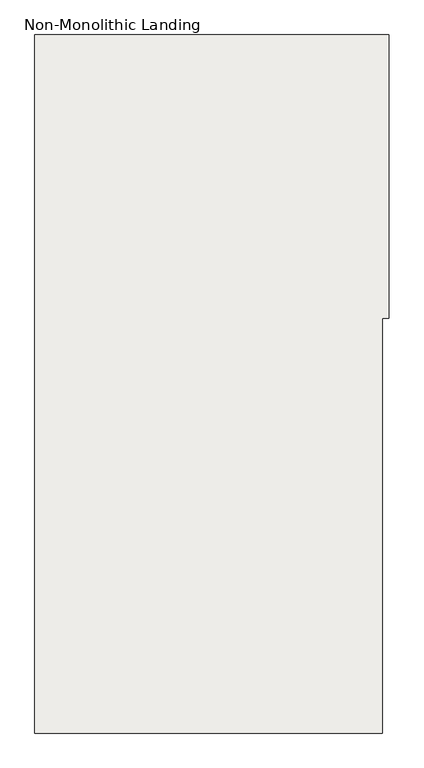
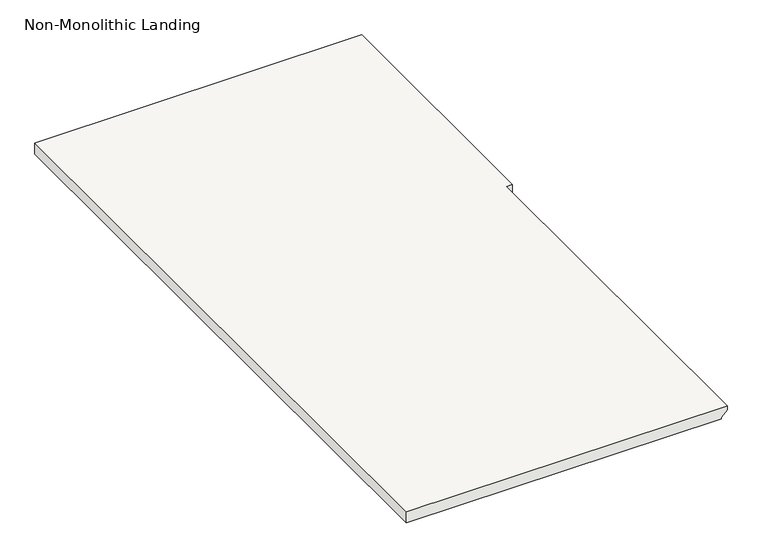
"""IFC4 building model written with IfcOpenShell, lengths in millimetres: slab geometry, Non-Monolithic Landing."""

from ifc_helpers import new_model, si_unit, origin, place, context, project, spatial, faceted_brep, source, transform, mapped, element, save


def non_monolithic_landing_cc7d3835(model_context):
    return source(origin(), model_context, "Body", "Brep", [
        faceted_brep([(-3502.6122732, 6497.5015304, 5554.4357143), (-3528.0122732, 6497.5015304, 5529.0357143), (-3528.0122732, 7615.1015304, 5529.0357143), (-3502.6122732, 7615.1015304, 5554.4357143), (-3502.6122732, 8132.6265304, 5573.4857143), (-3477.2122732, 8132.6265304, 5573.4857143), (-3477.2122732, 9250.2265304, 5573.4857143), (-3502.6122732, 9250.2265304, 5573.4857143), (-4874.2122732, 9250.2265304, 5573.4857143), (-4874.2122732, 6497.5015304, 5573.4857143), (-3502.6122732, 6497.5015304, 5573.4857143), (-3528.0122732, 7615.1015304, 5522.6857143), (-3528.0122732, 6497.5015304, 5522.6857143), (-4874.2122732, 6497.5015304, 5522.6857143), (-4874.2122732, 9250.2265304, 5522.6857143), (-3502.6122732, 9250.2265304, 5522.6857143), (-3477.2122732, 9250.2265304, 5522.6857143), (-3477.2122732, 8132.6265304, 5522.6857143), (-3502.6122732, 8132.6265304, 5522.6857143), (-3502.6122732, 7615.1015304, 5522.6857143)], [[[0, 1, 2, 3]], [[4, 5, 6, 7, 8, 9, 10]], [[11, 12, 13, 14, 15, 16, 17, 18, 19]], [[12, 11, 2, 1]], [[11, 19, 3, 2]], [[4, 10, 0, 3, 19, 18]], [[5, 4, 18, 17]], [[6, 5, 17, 16]], [[7, 6, 16, 15]], [[8, 7, 15, 14]], [[9, 8, 14, 13]], [[10, 9, 13, 12, 1, 0]]]),
    ])


if __name__ == "__main__":
    model = new_model("IFC4")
    model_context = context("Model", 3, world=origin())
    ifc_project = project(units=[si_unit("LENGTHUNIT", "METRE", prefix="MILLI")], contexts=[model_context])
    site = spatial("IfcSite", under=ifc_project)
    building = spatial("IfcBuilding", under=site)
    placement = place(None, origin())
    non_monolithic_landing_shape = non_monolithic_landing_cc7d3835(model_context)
    element("IfcSlab", 1, ObjectType="Non-Monolithic Landing", at=placement, inside=building, context=model_context, shape_type="MappedRepresentation", body=[
        mapped(non_monolithic_landing_shape, transform((0.0, 0.0, 0.0), x_axis=(1.0, 0.0, 0.0), y_axis=(0.0, 1.0, 0.0), z_axis=(0.0, 0.0, 1.0))),
    ])
    save(model, "model.ifc")
